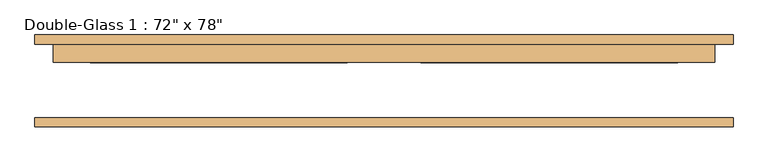
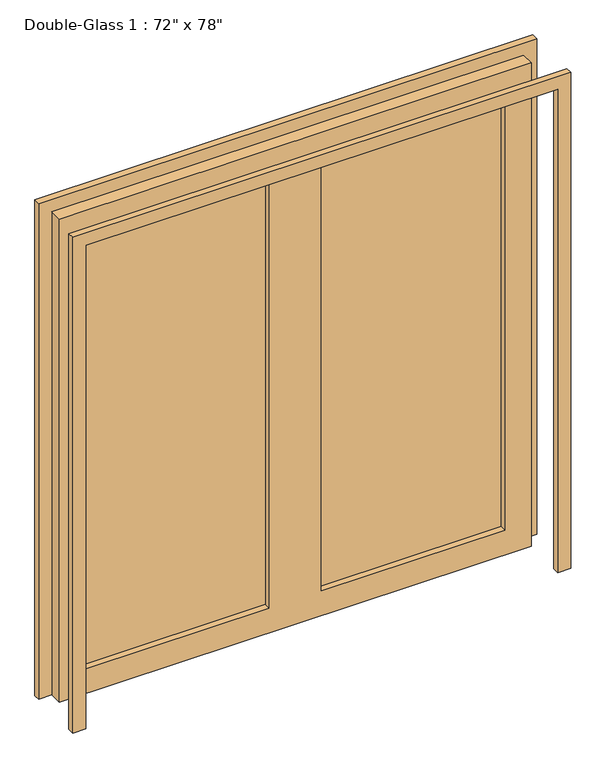
"""IFC4 building model written with IfcOpenShell, lengths in millimetres: door geometry."""

import ifcopenshell
import ifcopenshell.guid

model = None  # the IFC model being written
_history = None  # IfcOwnerHistory: only IFC2X3 demands one
_inside = {}  # id of a spatial element -> (the spatial element, [elements in it])
_under = {}  # id of a project, library or spatial element -> (it, [spatial elements below it])
_declared = {}  # id of a project -> (the project, [libraries it declares])
_typed = {}  # id of a type object -> (the type object, [elements of that type])
_made_of = {}  # id of a material, layer set ... -> (it, [elements and type objects made of it])


def new_model(schema):
    """Start an empty IFC model of exactly this schema.

    Asked for "IFC4X3", IfcOpenShell would pick the latest addendum, in which some entities
    have other attributes; the version numbers below select the first issue.
    IFC2X3 requires an IfcOwnerHistory on every rooted entity: one is made here for all.
    """
    global model, _history
    if schema == "IFC4X3":
        model = ifcopenshell.file(schema_version=(4, 3, 0, 0))
    else:
        model = ifcopenshell.file(schema=schema)
    _inside.clear()
    _under.clear()
    _declared.clear()
    _typed.clear()
    _made_of.clear()
    _history = None
    if model.schema == "IFC2X3":
        org = make("IfcOrganization", Name="unknown")
        user = make(
            "IfcPersonAndOrganization",
            ThePerson=make("IfcPerson", FamilyName="unknown"),
            TheOrganization=org,
        )
        app = make(
            "IfcApplication",
            ApplicationDeveloper=org,
            Version="unknown",
            ApplicationFullName="unknown",
            ApplicationIdentifier="unknown",
        )
        _history = make(
            "IfcOwnerHistory",
            OwningUser=user,
            OwningApplication=app,
            ChangeAction="ADDED",
            CreationDate=0,
        )
    return model


def make(cls, **values):
    """One entity of the class cls with the attributes given. An attribute that is None is left unset."""
    return model.create_entity(
        cls, **{name: value for name, value in values.items() if value is not None}
    )


def rooted(cls, **values):
    """An entity with a GlobalId (a new one), such as an element, a storey or a relation."""
    return make(cls, GlobalId=ifcopenshell.guid.new(), OwnerHistory=_history, **values)


def si_unit(unit_type, name, prefix=None):
    """IfcSIUnit, for example si_unit("LENGTHUNIT", "METRE", prefix="MILLI")."""
    return make("IfcSIUnit", UnitType=unit_type, Prefix=prefix, Name=name)


def assignment(units):
    """IfcUnitAssignment: the units of a project."""
    return None if units is None else make("IfcUnitAssignment", Units=units)


def point(xyz):
    """IfcCartesianPoint."""
    return None if xyz is None else make("IfcCartesianPoint", Coordinates=xyz)


def direction(xyz):
    """IfcDirection."""
    return None if xyz is None else make("IfcDirection", DirectionRatios=xyz)


def frame(location, z_axis=None, x_axis=None):
    """IfcAxis2Placement3D, a coordinate frame: its origin and axes. An axis left out is left unset."""
    return make(
        "IfcAxis2Placement3D",
        Location=point(location),
        Axis=direction(z_axis),
        RefDirection=direction(x_axis),
    )


def origin():
    """The frame at (0, 0, 0) with its axes left unset."""
    return frame((0.0, 0.0, 0.0))


def place(relative_to, where):
    """IfcLocalPlacement: puts the frame where relative to a parent placement (None: the world)."""
    return make(
        "IfcLocalPlacement", PlacementRelTo=relative_to, RelativePlacement=where
    )


def context(
    kind, dimensions, precision=None, world=None, true_north=None, identifier=None
):
    """IfcGeometricRepresentationContext, for example the 3D "Model" context."""
    return make(
        "IfcGeometricRepresentationContext",
        ContextIdentifier=identifier,
        ContextType=kind,
        CoordinateSpaceDimension=dimensions,
        Precision=precision,
        WorldCoordinateSystem=world,
        TrueNorth=true_north,
    )


def project(units=None, contexts=None):
    """IfcProject with its units and contexts."""
    return rooted(
        "IfcProject",
        Name="project",
        RepresentationContexts=contexts,
        UnitsInContext=assignment(units),
    )


def spatial(cls, under=None, at=None, **own):
    """A site, building, storey or space (cls), placed at a placement, below another one or the project."""
    s = rooted(cls, ObjectPlacement=at, **own)
    if under is not None:
        _under.setdefault(under.id(), (under, []))[1].append(s)
    return s


def polyline(points):
    """IfcPolyline through the points."""
    return make("IfcPolyline", Points=[point(p) for p in points])


def outline(outer, holes=None, kind="AREA"):
    """IfcArbitraryClosedProfileDef: a profile drawn as a closed curve; with holes, ...WithVoids."""
    if holes is None:
        return make("IfcArbitraryClosedProfileDef", ProfileType=kind, OuterCurve=outer)
    return make(
        "IfcArbitraryProfileDefWithVoids",
        ProfileType=kind,
        OuterCurve=outer,
        InnerCurves=holes,
    )


def extrude(swept, where, along, depth):
    """IfcExtrudedAreaSolid: the profile swept, set in the frame where, extruded along a direction by depth."""
    return make(
        "IfcExtrudedAreaSolid",
        SweptArea=swept,
        Position=where,
        ExtrudedDirection=direction(along),
        Depth=depth,
    )


def shape(context_of_items, identifier, shape_type, items):
    """IfcShapeRepresentation: the items that make up one representation, for example the "Body"."""
    return make(
        "IfcShapeRepresentation",
        ContextOfItems=context_of_items,
        RepresentationIdentifier=identifier,
        RepresentationType=shape_type,
        Items=items,
    )


def source(mapping_origin, context_of_items, identifier, shape_type, items):
    """IfcRepresentationMap: a shape defined once, which mapped items show again and again."""
    return make(
        "IfcRepresentationMap",
        MappingOrigin=mapping_origin,
        MappedRepresentation=shape(context_of_items, identifier, shape_type, items),
    )


def transform(
    local_origin,
    x_axis=None,
    y_axis=None,
    z_axis=None,
    scale=None,
    scale2=None,
    scale3=None,
    uniform=True,
):
    """IfcCartesianTransformationOperator3D, or its non-uniform kind. x_axis, y_axis, z_axis: its Axis1, 2, 3."""
    if uniform:
        return make(
            "IfcCartesianTransformationOperator3D",
            Axis1=direction(x_axis),
            Axis2=direction(y_axis),
            LocalOrigin=point(local_origin),
            Scale=scale,
            Axis3=direction(z_axis),
        )
    return make(
        "IfcCartesianTransformationOperator3DnonUniform",
        Axis1=direction(x_axis),
        Axis2=direction(y_axis),
        LocalOrigin=point(local_origin),
        Scale=scale,
        Axis3=direction(z_axis),
        Scale2=scale2,
        Scale3=scale3,
    )


def mapped(mapping_source, mapping_target):
    """IfcMappedItem: shows the shape of a source again, moved by a transform."""
    return make(
        "IfcMappedItem", MappingSource=mapping_source, MappingTarget=mapping_target
    )


def made_of(thing, what):
    """Note that an element or type object is made of a material, layer set ...; save() writes the relation."""
    if what is not None:
        _made_of.setdefault(what.id(), (what, []))[1].append(thing)
    return thing


def element(
    cls,
    number,
    at=None,
    inside=None,
    cuts=None,
    type_object=None,
    material=None,
    context=None,
    identifier="Body",
    shape_type=None,
    held_by="IfcProductDefinitionShape",
    body=None,
    shapes=None,
    **own,
):
    """One element of the class cls, such as IfcWall. Its Tag is "e" and its number.

    at: its placement. inside: the storey or other place that contains it. cuts: it is an
    opening in that element (IfcRelVoidsElement). A single representation is given by context,
    identifier, shape_type and body (its items); several are given by shapes. held_by: the class
    of the entity that holds the representations. save() writes the other relations.
    """
    e = rooted(cls, Tag="e%d" % number, ObjectPlacement=at, **own)
    if body is not None:
        shapes = [shape(context, identifier, shape_type, body)]
    if shapes is not None:
        e.Representation = make(held_by, Representations=shapes)
    if inside is not None:
        _inside.setdefault(inside.id(), (inside, []))[1].append(e)
    if cuts is not None:
        rooted(
            "IfcRelVoidsElement", RelatingBuildingElement=cuts, RelatedOpeningElement=e
        )
    if type_object is not None:
        _typed.setdefault(type_object.id(), (type_object, []))[1].append(e)
    return made_of(e, material)


def aggregate(whole, parts):
    """IfcRelAggregates: a whole, such as a stair, and the parts it consists of."""
    return rooted("IfcRelAggregates", RelatingObject=whole, RelatedObjects=parts)


def save(model, path):
    """Write the relations noted so far, then the file.

    IfcRelAggregates (storeys below a building ...), IfcRelContainedInSpatialStructure (elements
    in a storey), IfcRelDefinesByType, IfcRelAssociatesMaterial and IfcRelDeclares: one each for
    every whole, place, type object, material and project.
    """
    for whole, parts in _under.values():
        aggregate(whole, parts)
    for where, things in _inside.values():
        rooted(
            "IfcRelContainedInSpatialStructure",
            RelatedElements=things,
            RelatingStructure=where,
        )
    for kind, things in _typed.values():
        rooted("IfcRelDefinesByType", RelatedObjects=things, RelatingType=kind)
    for what, things in _made_of.values():
        rooted("IfcRelAssociatesMaterial", RelatedObjects=things, RelatingMaterial=what)
    for by, libraries in _declared.values():
        rooted("IfcRelDeclares", RelatingContext=by, RelatedDefinitions=libraries)
    model.write(path)


def door_5a05c884(model_context):
    return source(origin(), model_context, "Body", "SweptSolid", [
        extrude(outline(polyline([(0.0, 965.2), (2032.0, 965.2), (2032.0, -965.2), (0.0, -965.2), (0.0, -914.4), (1981.2, -914.4), (1981.2, 914.4), (0.0, 914.4), (0.0, 965.2)])), frame((0.0, -124.61875, 0.0), z_axis=(0.0, 1.0, 0.0), x_axis=(0.0, 0.0, 1.0)), (0.0, 0.0, 1.0), 25.4),
        extrude(outline(polyline([(1981.2, 914.4), (0.0, 914.4), (0.0, 965.2), (2032.0, 965.2), (2032.0, -965.2), (0.0, -965.2), (0.0, -914.4), (1981.2, -914.4), (1981.2, 914.4)])), frame((0.0, 103.98125, 0.0), z_axis=(0.0, 1.0, 0.0), x_axis=(0.0, 0.0, 1.0)), (0.0, 0.0, 1.0), 25.4),
        extrude(outline(polyline([(812.8, 78.58125), (101.6, 78.58125), (101.6, 85.725), (812.8, 85.725), (812.8, 78.58125)])), frame((0.0, 0.0, 101.6), z_axis=(0.0, 0.0, 1.0), x_axis=(1.0, 0.0, 0.0)), (0.0, 0.0, 1.0), 1778.0),
        extrude(outline(polyline([(-101.6, 78.58125), (-812.8, 78.58125), (-812.8, 85.725), (-101.6, 85.725), (-101.6, 78.58125)])), frame((0.0, 0.0, 101.6), z_axis=(0.0, 0.0, 1.0), x_axis=(1.0, 0.0, 0.0)), (0.0, 0.0, 1.0), 1778.0),
        extrude(outline(polyline([(1981.2, 914.4), (1981.2, -914.4), (0.0, -914.4), (0.0, 914.4), (1981.2, 914.4)]), holes=[polyline([(1879.6, -101.6), (101.6, -101.6), (101.6, -812.8), (1879.6, -812.8), (1879.6, -101.6)]), polyline([(1879.6, 812.8), (101.6, 812.8), (101.6, 101.6), (1879.6, 101.6), (1879.6, 812.8)])]), frame((0.0, 53.18125, 0.0), z_axis=(0.0, 1.0, 0.0), x_axis=(0.0, 0.0, 1.0)), (0.0, 0.0, 1.0), 50.8),
    ])


if __name__ == "__main__":
    model = new_model("IFC4")
    model_context = context("Model", 3, world=origin())
    ifc_project = project(units=[si_unit("LENGTHUNIT", "METRE", prefix="MILLI")], contexts=[model_context])
    site = spatial("IfcSite", under=ifc_project)
    building = spatial("IfcBuilding", under=site)
    placement = place(None, origin())
    door_shape = door_5a05c884(model_context)
    element("IfcDoor", 1, ObjectType="Double-Glass 1 : 72\" x 78\"", at=placement, inside=building, context=model_context, shape_type="MappedRepresentation", body=[
        mapped(door_shape, transform((0.0, 0.0, 0.0), x_axis=(1.0, 0.0, 0.0), y_axis=(0.0, 1.0, 0.0), z_axis=(0.0, 0.0, 1.0))),
    ])
    save(model, "model.ifc")

# Revit data of these elements
# Type "Double-Glass 1 : 72\" x 78\""
#   Type Mark = "32"
#   Assembly Code = "C1020"
#   Thickness = 0' - 2"
#   Height = 6' - 6"
#   Rail Width - Base = 0' - 4"
#   Rail Width - Top = 0' - 4"
#   Stile Width - Hinge = 0' - 4"
#   Stile Width - Latch = 0' - 4"
#   Trim Projection = 0' - 1"
#   Trim Width = 0' - 2"
#   Width = 6' - 0"
#   Define Thermal Properties by = 0
#   Function = 0
#   Door Material = Door - Panel
#   Frame Material = Door - Frame
#   Wall Closure = (empty or 0)
# Element 1 (IfcDoor, "Double-Glass 1 : 72\" x 78\"")
#   Materials on its faces: "Door - Frame", "Door - Panel", "Glass"
# Materials
#   "Door - Panel": class "Wood", colour RGB 227 170 128, transparency 0, Cost = 0
#   "Door - Frame": class "Miscellaneous", colour RGB 153 76 43, transparency 0, Cost = 0
#   "Glass": class "Glass", colour RGB 236 240 239, transparency 0.5, Description = "Soda Lime Glass", Cost = 0
